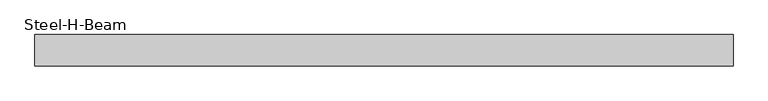
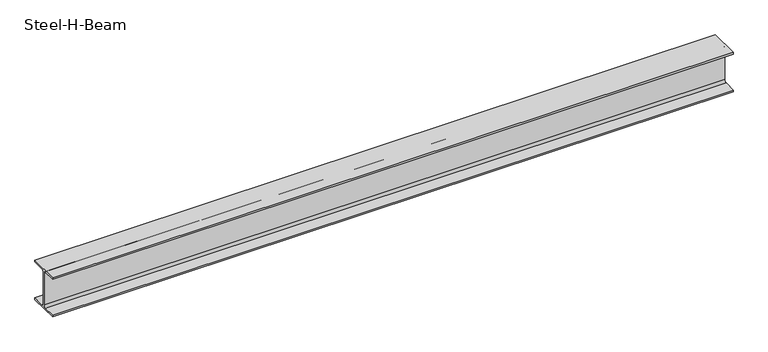
"""IFC4 building model written with IfcOpenShell, lengths in millimetres: beam geometry, Steel-H-Beam : BM121_H-340×250x9x14."""

import ifcopenshell
import ifcopenshell.guid

model = None  # the IFC model being written
_history = None  # IfcOwnerHistory: only IFC2X3 demands one
_inside = {}  # id of a spatial element -> (the spatial element, [elements in it])
_under = {}  # id of a project, library or spatial element -> (it, [spatial elements below it])
_declared = {}  # id of a project -> (the project, [libraries it declares])
_typed = {}  # id of a type object -> (the type object, [elements of that type])
_made_of = {}  # id of a material, layer set ... -> (it, [elements and type objects made of it])


def new_model(schema):
    """Start an empty IFC model of exactly this schema.

    Asked for "IFC4X3", IfcOpenShell would pick the latest addendum, in which some entities
    have other attributes; the version numbers below select the first issue.
    IFC2X3 requires an IfcOwnerHistory on every rooted entity: one is made here for all.
    """
    global model, _history
    if schema == "IFC4X3":
        model = ifcopenshell.file(schema_version=(4, 3, 0, 0))
    else:
        model = ifcopenshell.file(schema=schema)
    _inside.clear()
    _under.clear()
    _declared.clear()
    _typed.clear()
    _made_of.clear()
    _history = None
    if model.schema == "IFC2X3":
        org = make("IfcOrganization", Name="unknown")
        user = make(
            "IfcPersonAndOrganization",
            ThePerson=make("IfcPerson", FamilyName="unknown"),
            TheOrganization=org,
        )
        app = make(
            "IfcApplication",
            ApplicationDeveloper=org,
            Version="unknown",
            ApplicationFullName="unknown",
            ApplicationIdentifier="unknown",
        )
        _history = make(
            "IfcOwnerHistory",
            OwningUser=user,
            OwningApplication=app,
            ChangeAction="ADDED",
            CreationDate=0,
        )
    return model


def make(cls, **values):
    """One entity of the class cls with the attributes given. An attribute that is None is left unset."""
    return model.create_entity(
        cls, **{name: value for name, value in values.items() if value is not None}
    )


def rooted(cls, **values):
    """An entity with a GlobalId (a new one), such as an element, a storey or a relation."""
    return make(cls, GlobalId=ifcopenshell.guid.new(), OwnerHistory=_history, **values)


def si_unit(unit_type, name, prefix=None):
    """IfcSIUnit, for example si_unit("LENGTHUNIT", "METRE", prefix="MILLI")."""
    return make("IfcSIUnit", UnitType=unit_type, Prefix=prefix, Name=name)


def assignment(units):
    """IfcUnitAssignment: the units of a project."""
    return None if units is None else make("IfcUnitAssignment", Units=units)


def point(xyz):
    """IfcCartesianPoint."""
    return None if xyz is None else make("IfcCartesianPoint", Coordinates=xyz)


def direction(xyz):
    """IfcDirection."""
    return None if xyz is None else make("IfcDirection", DirectionRatios=xyz)


def frame(location, z_axis=None, x_axis=None):
    """IfcAxis2Placement3D, a coordinate frame: its origin and axes. An axis left out is left unset."""
    return make(
        "IfcAxis2Placement3D",
        Location=point(location),
        Axis=direction(z_axis),
        RefDirection=direction(x_axis),
    )


def frame_2d(location, x_axis=None):
    """IfcAxis2Placement2D, a coordinate frame in the plane: its origin and x axis."""
    return make(
        "IfcAxis2Placement2D", Location=point(location), RefDirection=direction(x_axis)
    )


def origin():
    """The frame at (0, 0, 0) with its axes left unset."""
    return frame((0.0, 0.0, 0.0))


def place(relative_to, where):
    """IfcLocalPlacement: puts the frame where relative to a parent placement (None: the world)."""
    return make(
        "IfcLocalPlacement", PlacementRelTo=relative_to, RelativePlacement=where
    )


def context(
    kind, dimensions, precision=None, world=None, true_north=None, identifier=None
):
    """IfcGeometricRepresentationContext, for example the 3D "Model" context."""
    return make(
        "IfcGeometricRepresentationContext",
        ContextIdentifier=identifier,
        ContextType=kind,
        CoordinateSpaceDimension=dimensions,
        Precision=precision,
        WorldCoordinateSystem=world,
        TrueNorth=true_north,
    )


def project(units=None, contexts=None):
    """IfcProject with its units and contexts."""
    return rooted(
        "IfcProject",
        Name="project",
        RepresentationContexts=contexts,
        UnitsInContext=assignment(units),
    )


def spatial(cls, under=None, at=None, **own):
    """A site, building, storey or space (cls), placed at a placement, below another one or the project."""
    s = rooted(cls, ObjectPlacement=at, **own)
    if under is not None:
        _under.setdefault(under.id(), (under, []))[1].append(s)
    return s


def polyline(points):
    """IfcPolyline through the points."""
    return make("IfcPolyline", Points=[point(p) for p in points])


def circle_curve(where, radius):
    """IfcCircle in the frame where."""
    return make("IfcCircle", Position=where, Radius=radius)


def trimmed(basis, trim1, trim2, sense, master):
    """IfcTrimmedCurve: the piece of a basis curve between two trims."""
    return make(
        "IfcTrimmedCurve",
        BasisCurve=basis,
        Trim1=trim1,
        Trim2=trim2,
        SenseAgreement=sense,
        MasterRepresentation=master,
    )


def segment(curve, same_sense, transition):
    """IfcCompositeCurveSegment."""
    return make(
        "IfcCompositeCurveSegment",
        Transition=transition,
        SameSense=same_sense,
        ParentCurve=curve,
    )


def composite_curve(segments, self_intersect=None):
    """IfcCompositeCurve: segments joined end to end."""
    return make("IfcCompositeCurve", Segments=segments, SelfIntersect=self_intersect)


def outline(outer, holes=None, kind="AREA"):
    """IfcArbitraryClosedProfileDef: a profile drawn as a closed curve; with holes, ...WithVoids."""
    if holes is None:
        return make("IfcArbitraryClosedProfileDef", ProfileType=kind, OuterCurve=outer)
    return make(
        "IfcArbitraryProfileDefWithVoids",
        ProfileType=kind,
        OuterCurve=outer,
        InnerCurves=holes,
    )


def extrude(swept, where, along, depth):
    """IfcExtrudedAreaSolid: the profile swept, set in the frame where, extruded along a direction by depth."""
    return make(
        "IfcExtrudedAreaSolid",
        SweptArea=swept,
        Position=where,
        ExtrudedDirection=direction(along),
        Depth=depth,
    )


def shape(context_of_items, identifier, shape_type, items):
    """IfcShapeRepresentation: the items that make up one representation, for example the "Body"."""
    return make(
        "IfcShapeRepresentation",
        ContextOfItems=context_of_items,
        RepresentationIdentifier=identifier,
        RepresentationType=shape_type,
        Items=items,
    )


def source(mapping_origin, context_of_items, identifier, shape_type, items):
    """IfcRepresentationMap: a shape defined once, which mapped items show again and again."""
    return make(
        "IfcRepresentationMap",
        MappingOrigin=mapping_origin,
        MappedRepresentation=shape(context_of_items, identifier, shape_type, items),
    )


def transform(
    local_origin,
    x_axis=None,
    y_axis=None,
    z_axis=None,
    scale=None,
    scale2=None,
    scale3=None,
    uniform=True,
):
    """IfcCartesianTransformationOperator3D, or its non-uniform kind. x_axis, y_axis, z_axis: its Axis1, 2, 3."""
    if uniform:
        return make(
            "IfcCartesianTransformationOperator3D",
            Axis1=direction(x_axis),
            Axis2=direction(y_axis),
            LocalOrigin=point(local_origin),
            Scale=scale,
            Axis3=direction(z_axis),
        )
    return make(
        "IfcCartesianTransformationOperator3DnonUniform",
        Axis1=direction(x_axis),
        Axis2=direction(y_axis),
        LocalOrigin=point(local_origin),
        Scale=scale,
        Axis3=direction(z_axis),
        Scale2=scale2,
        Scale3=scale3,
    )


def mapped(mapping_source, mapping_target):
    """IfcMappedItem: shows the shape of a source again, moved by a transform."""
    return make(
        "IfcMappedItem", MappingSource=mapping_source, MappingTarget=mapping_target
    )


def made_of(thing, what):
    """Note that an element or type object is made of a material, layer set ...; save() writes the relation."""
    if what is not None:
        _made_of.setdefault(what.id(), (what, []))[1].append(thing)
    return thing


def element(
    cls,
    number,
    at=None,
    inside=None,
    cuts=None,
    type_object=None,
    material=None,
    context=None,
    identifier="Body",
    shape_type=None,
    held_by="IfcProductDefinitionShape",
    body=None,
    shapes=None,
    **own,
):
    """One element of the class cls, such as IfcWall. Its Tag is "e" and its number.

    at: its placement. inside: the storey or other place that contains it. cuts: it is an
    opening in that element (IfcRelVoidsElement). A single representation is given by context,
    identifier, shape_type and body (its items); several are given by shapes. held_by: the class
    of the entity that holds the representations. save() writes the other relations.
    """
    e = rooted(cls, Tag="e%d" % number, ObjectPlacement=at, **own)
    if body is not None:
        shapes = [shape(context, identifier, shape_type, body)]
    if shapes is not None:
        e.Representation = make(held_by, Representations=shapes)
    if inside is not None:
        _inside.setdefault(inside.id(), (inside, []))[1].append(e)
    if cuts is not None:
        rooted(
            "IfcRelVoidsElement", RelatingBuildingElement=cuts, RelatedOpeningElement=e
        )
    if type_object is not None:
        _typed.setdefault(type_object.id(), (type_object, []))[1].append(e)
    return made_of(e, material)


def aggregate(whole, parts):
    """IfcRelAggregates: a whole, such as a stair, and the parts it consists of."""
    return rooted("IfcRelAggregates", RelatingObject=whole, RelatedObjects=parts)


def save(model, path):
    """Write the relations noted so far, then the file.

    IfcRelAggregates (storeys below a building ...), IfcRelContainedInSpatialStructure (elements
    in a storey), IfcRelDefinesByType, IfcRelAssociatesMaterial and IfcRelDeclares: one each for
    every whole, place, type object, material and project.
    """
    for whole, parts in _under.values():
        aggregate(whole, parts)
    for where, things in _inside.values():
        rooted(
            "IfcRelContainedInSpatialStructure",
            RelatedElements=things,
            RelatingStructure=where,
        )
    for kind, things in _typed.values():
        rooted("IfcRelDefinesByType", RelatedObjects=things, RelatingType=kind)
    for what, things in _made_of.values():
        rooted("IfcRelAssociatesMaterial", RelatedObjects=things, RelatingMaterial=what)
    for by, libraries in _declared.values():
        rooted("IfcRelDeclares", RelatingContext=by, RelatedDefinitions=libraries)
    model.write(path)


def steel_h_beam_3a09662f(model_context):
    return source(origin(), model_context, "Body", "SweptSolid", [
        extrude(outline(composite_curve([segment(polyline([(125.0, -156.0), (125.0, -170.0), (-125.0, -170.0), (-125.0, -156.0), (-24.5, -156.0)]), True, "CONTINUOUS"), segment(trimmed(circle_curve(frame_2d((-24.5, -136.0)), 20.0), [point((-24.5, -156.0))], [point((-4.5, -136.0))], True, "CARTESIAN"), True, "CONTINUOUS"), segment(polyline([(-4.5, -136.0), (-4.5, 136.0)]), True, "CONTINUOUS"), segment(trimmed(circle_curve(frame_2d((-24.5, 136.0)), 20.0), [point((-4.5, 136.0))], [point((-24.5, 156.0))], True, "CARTESIAN"), True, "CONTINUOUS"), segment(polyline([(-24.5, 156.0), (-125.0, 156.0), (-125.0, 170.0), (125.0, 170.0), (125.0, 156.0), (24.5, 156.0)]), True, "CONTINUOUS"), segment(trimmed(circle_curve(frame_2d((24.5, 136.0)), 20.0), [point((24.5, 156.0))], [point((4.5, 136.0))], True, "CARTESIAN"), True, "CONTINUOUS"), segment(polyline([(4.5, 136.0), (4.5, -136.0)]), True, "CONTINUOUS"), segment(trimmed(circle_curve(frame_2d((24.5, -136.0)), 20.0), [point((4.5, -136.0))], [point((24.5, -156.0))], True, "CARTESIAN"), True, "CONTINUOUS"), segment(polyline([(24.5, -156.0), (125.0, -156.0)]), True, "CONTINUOUS")], self_intersect=False)), frame((-2768.817822, 0.0, 0.0), z_axis=(1.0, 0.0, 0.0), x_axis=(0.0, 1.0, 0.0)), (0.0, 0.0, 1.0), 5580.2433846),
    ])


if __name__ == "__main__":
    model = new_model("IFC4")
    model_context = context("Model", 3, world=origin())
    ifc_project = project(units=[si_unit("LENGTHUNIT", "METRE", prefix="MILLI")], contexts=[model_context])
    site = spatial("IfcSite", under=ifc_project)
    building = spatial("IfcBuilding", under=site)
    placement = place(None, origin())
    steel_h_beam_shape = steel_h_beam_3a09662f(model_context)
    element("IfcBeam", 1, ObjectType="Steel-H-Beam : BM121_H-340×250x9x14", at=placement, inside=building, context=model_context, shape_type="MappedRepresentation", body=[
        mapped(steel_h_beam_shape, transform((0.0, 0.0, 0.0), x_axis=(1.0, 0.0, 0.0), y_axis=(0.0, 1.0, 0.0), z_axis=(0.0, 0.0, 1.0))),
    ])
    save(model, "model.ifc")

# Revit data of these elements
# Type "Steel-H-Beam : BM121_H-340×250x9x14"
#   Surface Area = 1.62766 m²/m
#   Section Area = 101.514 cm²
#   Mass per Unit Length = 79.6882 kg/m
#   Length [instance default] = 3000 mm
#   B = 250 mm
#   H = 340 mm
#   r = 20 mm
#   tw = 9 mm
#   tf = 14 mm
#   hec_material4 [instance default] = none
#   hec_material3 [instance default] = none
#   hec_material2 [instance default] = none
#   hec_material1 [instance default] = none
#   Structural Material [instance default] = Steel, 45-345
#   Assembly Code = ""
# Element 1 (IfcBeam, "Steel-H-Beam : BM121_H-340×250x9x14")
#   hec_material4 = S01AA010-00002_Main Steel Structure Fabrication Work_Shelter/Building_Steel Painting/Coating_for Fireproofed Steel Surface, Surface Preparation & Primer Coat
#   hec_material3 = F01AC000-00002_Building/Shelter Fire Proofing Work_Intumescent Coating Type_1 hr. rating (UL 1709))
#   hec_material2 = S01AA010-00002_Main Steel Structure Fabrication Work_Shelter/Building_Steel Painting/Coating_for Fireproofed Steel Surface, Surface Preparation & Primer Coat
#   hec_material1 = S03AA028-00001_Main Steel Structure Erection Work_Shelter/Building_Medium Steel
#   Structural Material = S01AA002-00001_Main Steel Structure Fabrication Work_Shelter/Building_Medium Steel - Standard
#   Materials on its faces: "S01AA002-00001_Main Steel Structure Fabrication Work_Shelter/Building_Medium Steel - Standard"
# Materials
#   "Steel, 45-345": class "Metal", colour RGB 189 187 185, transparency 0, Description = "Steel 345 MPa", Cost = 0
#   "S01AA002-00001_Main Steel Structure Fabrication Work_Shelter/Building_Medium Steel - Standard": class "Metal", colour RGB 120 120 120, transparency 0, Comments = "(90KG/M>Weight≥30KG/M)", Description = "Structural steel 50ksi", W00) Work Master Code = "S01AA002-0001", W01) Work Master_Lv1 = "Main Steel Structure Fabrication Work", W02) Work Master_Lv2 = "Shelter/Building", W03) Work Master_Spec.1 = "Medium Steel - Standard (90KG/M>Weight≥30KG/M)", Cost = 0
#   "S01AA010-00002_Main Steel Structure Fabrication Work_Shelter/Building_Steel Painting/Coating_for Fireproofed Steel Surface, Surface Preparation & Primer Coat": class "Metal", colour RGB 120 120 120, transparency 0, Description = "Paint finished steel", W00) Work Master Code = "SS01AA010-00002", W01) Work Master_Lv1 = "Main Steel Structure Fabrication Work", W02) Work Master_Lv2 = "Shelter/Building", W03) Work Master_Spec.1 = "Steel Painting/Coating", W04) Work Master_Spec.2 = "for Fireproofed Steel Surface, Surface Preparation & Primer Coat", Cost = 0
#   "F01AC000-00002_Building/Shelter Fire Proofing Work_Intumescent Coating Type_1 hr. rating (UL 1709))": class "Metal", colour RGB 255 128 128, transparency 0, Description = "Paint finished steel", W00) Work Master Code = "F01AC000-00002", W01) Work Master_Lv1 = "Building/Shelter Fire Proofing Work", W02) Work Master_Lv2 = "Intumescent Coating Type", W03) Work Master_Spec.1 = "1 hr. rating (UL 1709)", Cost = 0
#   "S03AA028-00001_Main Steel Structure Erection Work_Shelter/Building_Medium Steel": class "Metal", colour RGB 120 120 120, transparency 0, Comments = "(90KG/M>Weight≥30KG/M)", Description = "Structural steel 50ksi", W00) Work Master Code = "S03AA028-0001", W01) Work Master_Lv1 = "Main Steel Structure Erection Work", W02) Work Master_Lv2 = "Shelter/Building", W03) Work Master_Spec.1 = "Medium Steel (90KG/M>Weight≥30KG/M)", Cost = 0
